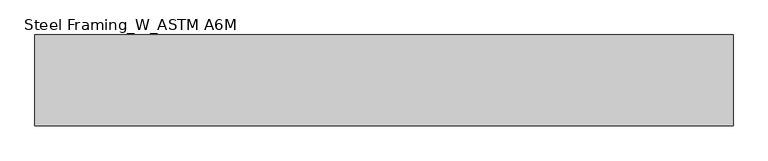
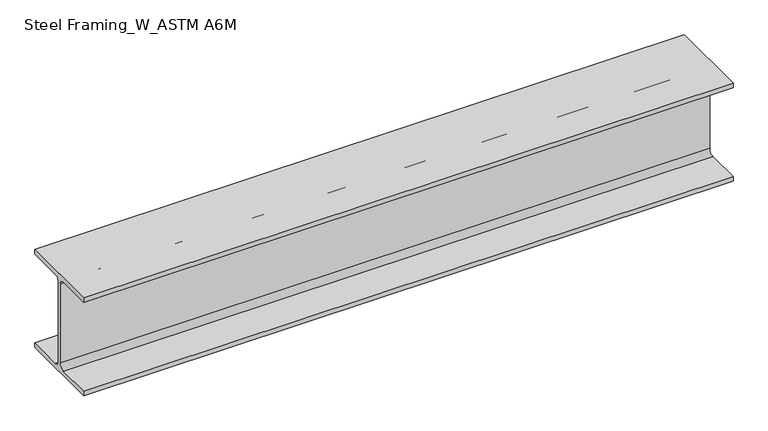
"""IFC4 building model written with IfcOpenShell, lengths in millimetres: beam geometry, Steel Framing_W_ASTM A6M : H_SB_AR_S02_W250x49.1_G5."""

from ifc_helpers import new_model, si_unit, point, frame, frame_2d, origin, place, context, project, spatial, polyline, circle_curve, trimmed, segment, composite_curve, outline, extrude, source, transform, mapped, element, save


def steel_framing_w_astm_a6m_56f27783(model_context):
    return source(origin(), model_context, "Body", "SweptSolid", [
        extrude(outline(composite_curve([segment(polyline([(101.0, -112.5), (101.0, -123.5), (-101.0, -123.5), (-101.0, -112.5), (-16.385, -112.5)]), True, "CONTINUOUS"), segment(trimmed(circle_curve(frame_2d((-16.385, -99.8)), 12.7), [point((-16.385, -112.5))], [point((-3.685, -99.8))], True, "CARTESIAN"), True, "CONTINUOUS"), segment(polyline([(-3.685, -99.8), (-3.685, 99.8)]), True, "CONTINUOUS"), segment(trimmed(circle_curve(frame_2d((-16.385, 99.8)), 12.7), [point((-3.685, 99.8))], [point((-16.385, 112.5))], True, "CARTESIAN"), True, "CONTINUOUS"), segment(polyline([(-16.385, 112.5), (-101.0, 112.5), (-101.0, 123.5), (101.0, 123.5), (101.0, 112.5), (16.385, 112.5)]), True, "CONTINUOUS"), segment(trimmed(circle_curve(frame_2d((16.385, 99.8)), 12.7), [point((16.385, 112.5))], [point((3.685, 99.8))], True, "CARTESIAN"), True, "CONTINUOUS"), segment(polyline([(3.685, 99.8), (3.685, -99.8)]), True, "CONTINUOUS"), segment(trimmed(circle_curve(frame_2d((16.385, -99.8)), 12.7), [point((3.685, -99.8))], [point((16.385, -112.5))], True, "CARTESIAN"), True, "CONTINUOUS"), segment(polyline([(16.385, -112.5), (101.0, -112.5)]), True, "CONTINUOUS")], self_intersect=False)), frame((-684.3, 0.0, 0.0), z_axis=(1.0, 0.0, 0.0), x_axis=(0.0, 1.0, 0.0)), (0.0, 0.0, 1.0), 1551.3),
    ])


if __name__ == "__main__":
    model = new_model("IFC4")
    model_context = context("Model", 3, world=origin())
    ifc_project = project(units=[si_unit("LENGTHUNIT", "METRE", prefix="MILLI")], contexts=[model_context])
    site = spatial("IfcSite", under=ifc_project)
    building = spatial("IfcBuilding", under=site)
    placement = place(None, origin())
    steel_framing_w_astm_a6m_shape = steel_framing_w_astm_a6m_56f27783(model_context)
    element("IfcBeam", 1, ObjectType="Steel Framing_W_ASTM A6M : H_SB_AR_S02_W250x49.1_G5", at=placement, inside=building, context=model_context, shape_type="MappedRepresentation", body=[
        mapped(steel_framing_w_astm_a6m_shape, transform((0.0, 0.0, 0.0), x_axis=(1.0, 0.0, 0.0), y_axis=(0.0, 1.0, 0.0), z_axis=(0.0, 0.0, 1.0))),
    ])
    save(model, "model.ifc")

# Revit data of these elements
# Type "Steel Framing_W_ASTM A6M : H_SB_AR_S02_W250x49.1_G5"
#   Type Mark = "G5"
#   Section Name Key = "W10x33"
#   Width = 20.2 cm
#   Web Thickness = 0.737 cm
#   Web Fillet = 1.27 cm
#   Warping Constant = 212000.0 cm⁶
#   Torsional Moment of Inertia = 24.30 cm⁴
#   Section Area = 62.6 cm²
#   Plastic Modulus weak axis = 229.0 cm³
#   Plastic Modulus strong axis = 636.0 cm³
#   Perimeter = 1.27 m²/m
#   Nominal Weight = 49.10 kgf/m
#   Moment of Inertia weak axis = 1520.00 cm⁴
#   Moment of Inertia strong axis = 7120.00 cm⁴
#   Height = 24.7 cm
#   Flange Thickness = 1.1 cm
#   Elastic Modulus weak axis = 151.0 cm³
#   Elastic Modulus strong axis = 574.0 cm³
#   Centroid Vertical = 12.35 cm
#   Centroid Horizontal = 10.1 cm
#   Length [instance default] = 1500 mm
#   Structural Material [instance default] = Steel, 45-345
#   Bolt Spacing = 0
#   Assembly Code = ""
# Element 1 (IfcBeam, "Steel Framing_W_ASTM A6M : H_SB_AR_S02_W250x49.1_G5")
#   Materials on its faces: "Steel, 45-345"
# Materials
#   "Steel, 45-345": class "Metal", colour RGB 189 187 185, transparency 0, Description = "Steel 345 MPa", Cost = 0
